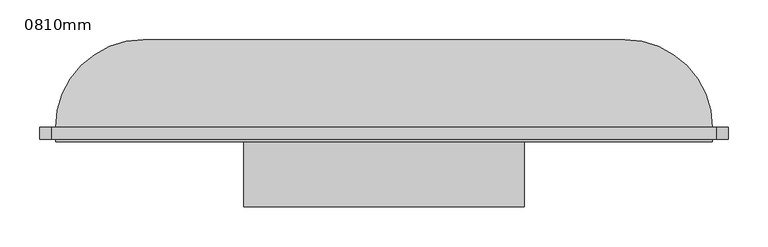
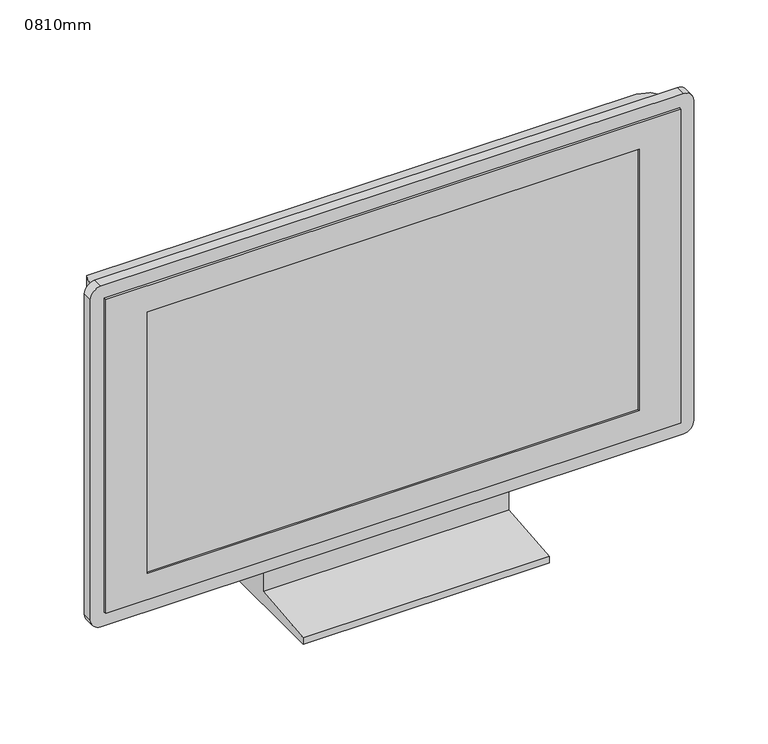
"""IFC4 building model written with IfcOpenShell, lengths in millimetres: proxy geometry, 电视 - 平板 : 0810mm."""

from ifc_helpers import new_model, si_unit, point, frame, frame_2d, origin, place, context, project, spatial, polyline, circle_curve, ellipse_curve, trimmed, segment, composite_curve, outline, extrude, faceted_brep, source, transform, mapped, element, save
from ifc_brep_helpers import plane_surface, cylinder_surface, advanced_brep


def proxy_0810mm_56245f3a(model_context):
    return source(origin(), model_context, "Body", "SolidModel", [
        extrude(outline(polyline([(-51.4613764, 80.0), (-1.4613764, 80.0), (48.5386236, 0.0), (-151.4613764, 0.0), (-151.4613764, 10.0), (-51.4613764, 20.0), (-51.4613764, 80.0)])), frame((-180.4346678, 0.0, 0.0), z_axis=(1.0, 0.0, 0.0), x_axis=(0.0, 1.0, 0.0)), (0.0, 0.0, 1.0), 352.9803073),
        faceted_brep([(409.0357931, -69.4613764, 557.1392838), (-416.9248214, -69.4613764, 557.1392838), (-416.9248214, -69.4613764, 80.0), (409.0357931, -69.4613764, 80.0), (-356.9248214, -69.4613764, 517.1392838), (349.0357931, -69.4613764, 517.1392838), (349.0357931, -69.4613764, 120.0), (-356.9248214, -69.4613764, 120.0), (409.0357931, -51.4613764, 557.1392838), (409.0357931, -51.4613764, 80.0), (-416.9248214, -51.4613764, 80.0), (-416.9248214, -51.4613764, 557.1392838), (-356.9248214, -66.4613764, 517.1392838), (-356.9248214, -66.4613764, 120.0), (349.0357931, -66.4613764, 120.0), (349.0357931, -66.4613764, 517.1392838)], [[[0, 1, 2, 3], [4, 5, 6, 7]], [[8, 9, 10, 11]], [[1, 0, 8, 11]], [[2, 1, 11, 10]], [[3, 2, 10, 9]], [[0, 3, 9, 8]], [[12, 13, 14, 15]], [[12, 15, 5, 4]], [[15, 14, 6, 5]], [[14, 13, 7, 6]], [[13, 12, 4, 7]]]),
        extrude(outline(composite_curve([segment(polyline([(577.1392838, 414.0357931), (577.1392838, -421.9248214)]), True, "CONTINUOUS"), segment(trimmed(circle_curve(frame_2d((562.1392838, -421.9248214)), 15.0), [point((577.1392838, -421.9248214))], [point((562.1392838, -436.9248214))], False, "CARTESIAN"), True, "CONTINUOUS"), segment(polyline([(562.1392838, -436.9248214), (75.0, -436.9248214)]), True, "CONTINUOUS"), segment(trimmed(circle_curve(frame_2d((75.0, -421.9248214)), 15.0), [point((75.0, -436.9248214))], [point((60.0, -421.9248214))], False, "CARTESIAN"), True, "CONTINUOUS"), segment(polyline([(60.0, -421.9248214), (60.0, 414.0357931)]), True, "CONTINUOUS"), segment(trimmed(circle_curve(frame_2d((75.0, 414.0357931)), 15.0), [point((60.0, 414.0357931))], [point((75.0, 429.0357931))], False, "CARTESIAN"), True, "CONTINUOUS"), segment(polyline([(75.0, 429.0357931), (562.1392838, 429.0357931)]), True, "CONTINUOUS"), segment(trimmed(circle_curve(frame_2d((562.1392838, 414.0357931)), 15.0), [point((562.1392838, 429.0357931))], [point((577.1392838, 414.0357931))], False, "CARTESIAN"), True, "CONTINUOUS")], self_intersect=False), holes=[polyline([(557.1392838, 409.0357931), (80.0, 409.0357931), (80.0, -416.9248214), (557.1392838, -416.9248214), (557.1392838, 409.0357931)])]), frame((0.0, -66.4613764, 0.0), z_axis=(0.0, 1.0, 0.0), x_axis=(0.0, 0.0, 1.0)), (0.0, 0.0, 1.0), 15.0),
        advanced_brep(
        [(-416.9248214, -51.4613764, 80.0), (409.0357931, -51.4613764, 80.0), (409.0357931, -51.4613764, 557.1392838), (-416.9248214, -51.4613764, 557.1392838), (299.0357931, 58.5386236, 80.0), (-306.9248214, 58.5386236, 80.0), (-306.9248214, 58.5386236, 447.1392838), (299.0357931, 58.5386236, 447.1392838)],
        [
            (0, 1),
            (1, 2),
            (2, 3),
            (3, 0),
            (4, 5),
            (5, 6),
            (6, 7),
            (7, 4),
            (0, 5, circle_curve(frame((-306.9248214, -51.4613764, 80.0), z_axis=(0.0, 0.0, -1.0), x_axis=(-1.0, 0.0, 0.0)), 110.0)),
            (4, 1, circle_curve(frame((299.0357931, -51.4613764, 80.0), z_axis=(0.0, 0.0, -1.0), x_axis=(1.0, 0.0, 0.0)), 110.0)),
            (7, 2, ellipse_curve(frame((299.0357931, -51.4613764, 447.1392838), z_axis=(0.7071067811865475, 0.0, -0.7071067811865475), x_axis=(0.7071067811865474, 0.0, 0.7071067811865476)), 155.5634919, 110.0)),
            (6, 3, ellipse_curve(frame((-306.9248214, -51.4613764, 447.1392838), z_axis=(0.7071067811865475, 0.0, 0.7071067811865475), x_axis=(-0.7071067811865476, 0.0, 0.7071067811865474)), 155.5634919, 110.0)),
        ],
        [
            plane_surface(frame((-416.9248214, -51.4613764, 557.1392838), z_axis=(0.0, -1.0, 0.0), x_axis=(-1.0, 0.0, 0.0))),
            plane_surface(frame((-416.9248214, 58.5386236, 557.1392838), z_axis=(0.0, 1.0, 0.0), x_axis=(1.0, 0.0, 0.0))),
            plane_surface(frame((-416.9248214, -51.4613764, 80.0), z_axis=(0.0, 0.0, -1.0), x_axis=(0.0, 1.0, 0.0))),
            cylinder_surface(frame((299.0357931, -51.4613764, 80.0), z_axis=(0.0, 0.0, 1.0), x_axis=(1.0, 0.0, 0.0)), 110.0),
            cylinder_surface(frame((409.0357931, -51.4613764, 447.1392838), z_axis=(-1.0, 0.0, 0.0), x_axis=(0.0, 0.0, 1.0)), 110.0),
            cylinder_surface(frame((-306.9248214, -51.4613764, 557.1392838), z_axis=(0.0, 0.0, -1.0), x_axis=(-1.0, 0.0, 0.0)), 110.0),
        ],
        [
            (0, [[1, 2, 3, 4]]),
            (1, [[5, 6, 7, 8]]),
            (2, [[-1, 9, -5, 10]]),
            (3, [[11, -2, -10, -8]]),
            (4, [[-11, -7, 12, -3]]),
            (5, [[-12, -6, -9, -4]]),
        ],
    ),
    ])


if __name__ == "__main__":
    model = new_model("IFC4")
    model_context = context("Model", 3, world=origin())
    ifc_project = project(units=[si_unit("LENGTHUNIT", "METRE", prefix="MILLI")], contexts=[model_context])
    site = spatial("IfcSite", under=ifc_project)
    building = spatial("IfcBuilding", under=site)
    placement = place(None, origin())
    proxy_0810mm_shape = proxy_0810mm_56245f3a(model_context)
    element("IfcBuildingElementProxy", 1, Name="电视 - 平板 : 0810mm", ObjectType="电视 - 平板 : 0810mm", at=placement, inside=building, context=model_context, shape_type="MappedRepresentation", body=[
        mapped(proxy_0810mm_shape, transform((0.0, 0.0, 0.0), x_axis=(1.0, 0.0, 0.0), y_axis=(0.0, 1.0, 0.0), z_axis=(0.0, 0.0, 1.0))),
    ])
    save(model, "model.ifc")

# Revit data of these elements
# Type "电视 - 平板 : 0810mm"
#   SinAng = 0.49 mm
#   L = 705.961 mm
#   H = 397.139 mm
#   厚度 = 110 mm
#   对角线 = 810 mm
#   CosAng = 0.872 mm
#   支架 [instance default] = yes
# Element 1 (IfcBuildingElementProxy, "电视 - 平板 : 0810mm")
#   Materials on its faces: "电视 - 黑色", "电视 - 玻璃", "电视 - 屏幕"
# Materials
#   "电视 - 黑色": class "其他", colour RGB 49 49 49, transparency 0
#   "电视 - 玻璃": class "其他", colour RGB 157 157 157, transparency 0.9
#   "电视 - 屏幕": class "其他", colour RGB 0 0 0, transparency 0
